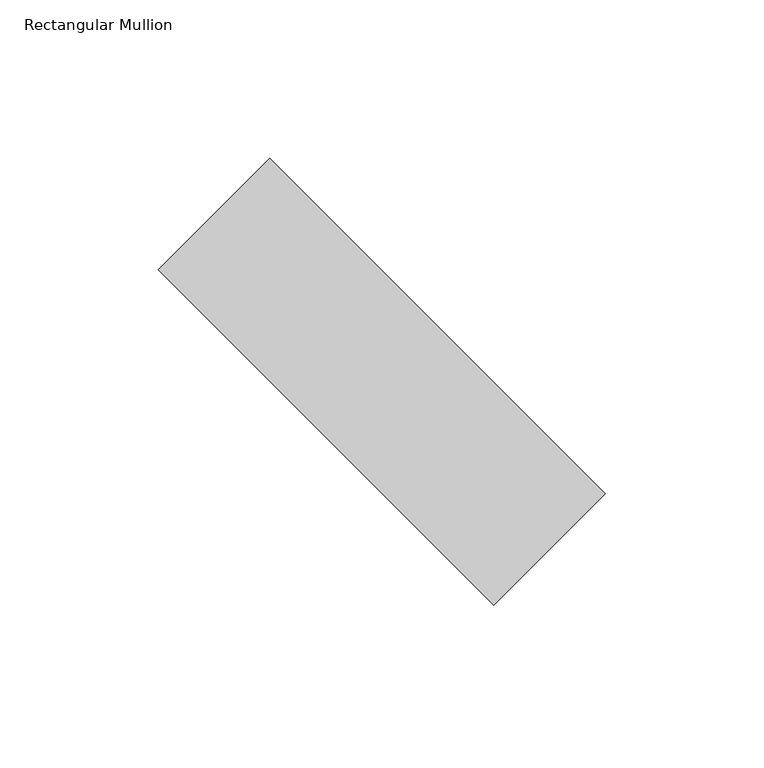
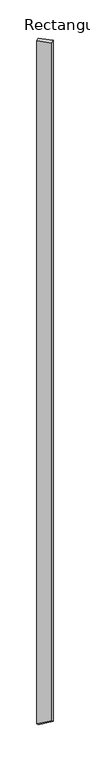
"""IFC4 building model written with IfcOpenShell, lengths in millimetres: member geometry, Rectangular Mullion : tilted mullions."""

from ifc_helpers import new_model, si_unit, origin, place, context, project, spatial, faceted_brep, source, transform, mapped, element, save


def rectangular_mullion_58c31241(model_context):
    return source(origin(), model_context, "Body", "Brep", [
        faceted_brep([(-35.3553391, 70.7106781, 0.0), (-70.7106781, 35.3553391, 0.0), (35.3553391, -70.7106781, 0.0), (70.7106781, -35.3553391, 0.0), (-35.3553391, 70.7106781, -8054.8135818), (-70.7106781, 35.3553391, -8009.8139729), (35.3553391, -70.7106781, -7944.4280666), (70.7106781, -35.3553391, -7989.4276756)], [[[0, 1, 2, 3]], [[1, 0, 4, 5]], [[2, 1, 5, 6]], [[3, 2, 6, 7]], [[0, 3, 7, 4]], [[4, 7, 6, 5]]]),
    ])


if __name__ == "__main__":
    model = new_model("IFC4")
    model_context = context("Model", 3, world=origin())
    ifc_project = project(units=[si_unit("LENGTHUNIT", "METRE", prefix="MILLI")], contexts=[model_context])
    site = spatial("IfcSite", under=ifc_project)
    building = spatial("IfcBuilding", under=site)
    placement = place(None, origin())
    rectangular_mullion_shape = rectangular_mullion_58c31241(model_context)
    element("IfcMember", 1, ObjectType="Rectangular Mullion : tilted mullions", at=placement, inside=building, context=model_context, shape_type="MappedRepresentation", body=[
        mapped(rectangular_mullion_shape, transform((0.0, 0.0, 0.0), x_axis=(1.0, 0.0, 0.0), y_axis=(0.0, 1.0, 0.0), z_axis=(0.0, 0.0, 1.0))),
    ])
    save(model, "model.ifc")

# Revit data of these elements
# Type "Rectangular Mullion : tilted mullions"
#   built-in parameter 1007304 = 0.492126 (stored number, unit not read)
#   built-in parameter 1007301 = 0.082021 (stored number, unit not read)
#   built-in parameter 1007300 = 0.082021 (stored number, unit not read)
# Element 1 (IfcMember, "Rectangular Mullion : tilted mullions")
#   Materials on its faces: "Aluminum"
# Materials
#   "Aluminum": class "Metal", colour RGB 244 244 244, transparency 0, Description = "Aluminum 6061", Cost = 0
